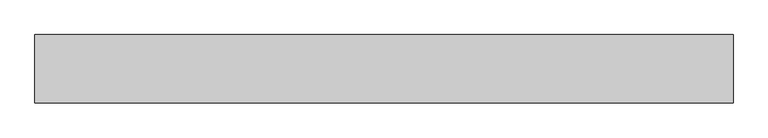
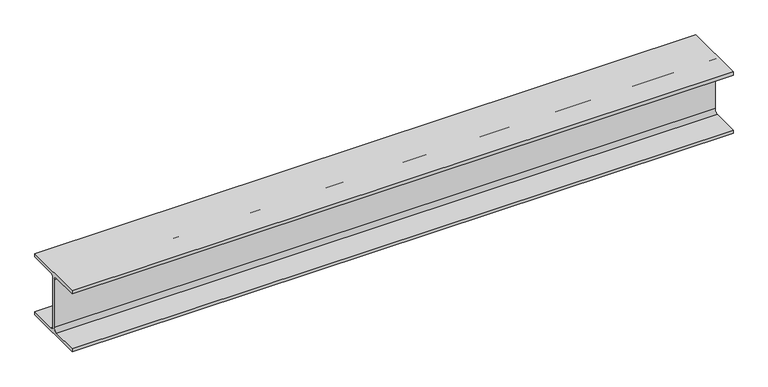
"""IFC4 building model written with IfcOpenShell, lengths in millimetres: beam geometry, 0912_Steel Framing_H-KSD3502 : H_SB_ASB_H-300x300x10x15."""

from ifc_helpers import new_model, si_unit, point, frame, frame_2d, origin, place, context, project, spatial, polyline, circle_curve, trimmed, segment, composite_curve, outline, extrude, source, transform, mapped, element, save


def beam_a9f46486(model_context):
    return source(origin(), model_context, "Body", "SweptSolid", [
        extrude(outline(composite_curve([segment(polyline([(150.0, -135.0), (150.0, -150.0), (-150.0, -150.0), (-150.0, -135.0), (-23.0, -135.0)]), True, "CONTINUOUS"), segment(trimmed(circle_curve(frame_2d((-23.0, -117.0)), 18.0), [point((-23.0, -135.0))], [point((-5.0, -117.0))], True, "CARTESIAN"), True, "CONTINUOUS"), segment(polyline([(-5.0, -117.0), (-5.0, 117.0)]), True, "CONTINUOUS"), segment(trimmed(circle_curve(frame_2d((-23.0, 117.0)), 18.0), [point((-5.0, 117.0))], [point((-23.0, 135.0))], True, "CARTESIAN"), True, "CONTINUOUS"), segment(polyline([(-23.0, 135.0), (-150.0, 135.0), (-150.0, 150.0), (150.0, 150.0), (150.0, 135.0), (23.0, 135.0)]), True, "CONTINUOUS"), segment(trimmed(circle_curve(frame_2d((23.0, 117.0)), 18.0), [point((23.0, 135.0))], [point((5.0, 117.0))], True, "CARTESIAN"), True, "CONTINUOUS"), segment(polyline([(5.0, 117.0), (5.0, -117.0)]), True, "CONTINUOUS"), segment(trimmed(circle_curve(frame_2d((23.0, -117.0)), 18.0), [point((5.0, -117.0))], [point((23.0, -135.0))], True, "CARTESIAN"), True, "CONTINUOUS"), segment(polyline([(23.0, -135.0), (150.0, -135.0)]), True, "CONTINUOUS")], self_intersect=False)), frame((-1364.2332089, 0.0, 0.0), z_axis=(1.0, 0.0, 0.0), x_axis=(0.0, 1.0, 0.0)), (0.0, 0.0, 1.0), 3068.3751225),
    ])


if __name__ == "__main__":
    model = new_model("IFC4")
    model_context = context("Model", 3, world=origin())
    ifc_project = project(units=[si_unit("LENGTHUNIT", "METRE", prefix="MILLI")], contexts=[model_context])
    site = spatial("IfcSite", under=ifc_project)
    building = spatial("IfcBuilding", under=site)
    placement = place(None, origin())
    beam_shape = beam_a9f46486(model_context)
    element("IfcBeam", 1, ObjectType="0912_Steel Framing_H-KSD3502 : H_SB_ASB_H-300x300x10x15", at=placement, inside=building, context=model_context, shape_type="MappedRepresentation", body=[
        mapped(beam_shape, transform((0.0, 0.0, 0.0), x_axis=(1.0, 0.0, 0.0), y_axis=(0.0, 1.0, 0.0), z_axis=(0.0, 0.0, 1.0))),
    ])
    save(model, "model.ifc")

# Revit data of these elements
# Type "0912_Steel Framing_H-KSD3502 : H_SB_ASB_H-300x300x10x15"
#   H_WM Code_1 = "S01AA001-00001 | Main Steel Structure Fabrication Work | Shelter/Building | Heavy Steel - Standard (Weight≥90KG/M) | Material: (   )"
#   H_WM Code_2 = "S03AA027-00001 | Main Steel Structure Erection Work | Shelter/Building | Heavy Steel (Weight≥90KG/M) | Material: (   )"
#   H_WM Code_3 = "S01AA010-00001 | Main Steel Structure Fabrication Work | Shelter/Building | Steel Painting/Coating | for Non-Fireproofed Steel Surface, Surface Preparation, Primer, Second & Final Coat | Material: (   )"
#   H_Q'ty Cal Type Tag = "SB-Q2"
#   Width = 30.0 cm
#   Web Thickness = 1.0 cm
#   Web Fillet = 1.8 cm
#   Warping Constant = 1370000.0 cm⁶
#   W = 0
#   Torsional Moment of Inertia = 77.00 cm⁴
#   Section Area = 119.8 cm²
#   Plastic Modulus weak axis = 684.0 cm³
#   Plastic Modulus strong axis = 1500.0 cm³
#   Perimeter = 1.75 m²/m
#   Nominal Weight = 94.00 kgf/m
#   Moment of Inertia weak axis = 6750.00 cm⁴
#   Moment of Inertia strong axis = 20400.00 cm⁴
#   Height = 30.0 cm
#   Flange Thickness = 1.5 cm
#   Elastic Modulus weak axis = 450.0 cm³
#   Elastic Modulus strong axis = 1360.0 cm³
#   Centroid Vertical = 15.0 cm
#   Centroid Horizontal = 15.0 cm
#   Ix = 204000000
#   Length [instance default] = 1.5240 m
#   Zx = 1500000
#   b = 0.3000 m
#   h = 0.3000 m
#   r = 0.0180 m
#   s = 0.0100 m
#   t = 0.0150 m
#   A = 0.01198 m²
#   Structural Material [instance default] = Steel, 45-345
#   Assembly Code = ""
# Element 1 (IfcBeam, "0912_Steel Framing_H-KSD3502 : H_SB_ASB_H-300x300x10x15")
#   Structural Material = none
# Materials
#   "Steel, 45-345": class "Metal", colour RGB 189 187 185, transparency 0, Description = "Steel 345 MPa", Cost = 0
